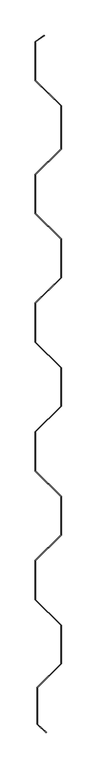
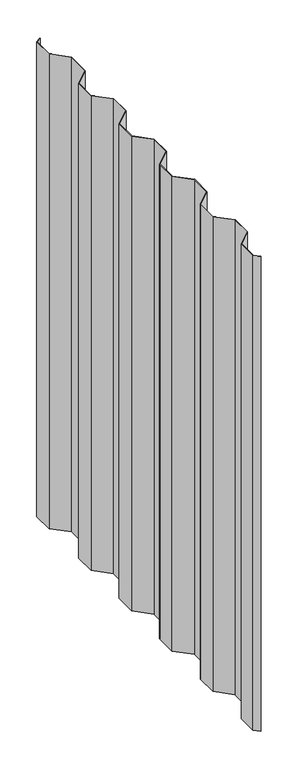
"""IFC4 building model written with IfcOpenShell, lengths in millimetres: proxy geometry, Generic Models 2:Generic Models 2:310765:Generic Models 2:310765 : Generic Models 2:Generic Models 2:310765:196 : Generic Models 2:Generic Models 2:310765:Generic Models 2:310765 : Generic Models 2:Generic Models 2:310765:300385."""

from ifc_helpers import new_model, si_unit, frame, origin, place, context, project, spatial, polyline, outline, extrude, source, transform, mapped, element, save


def generic_models_bcbc0872(model_context):
    return source(origin(), model_context, "Body", "SweptSolid", [
        extrude(outline(polyline([(579050.1098867, -578737.8387429), (579050.1098867, -578685.2449371), (579084.6679739, -578651.6129524), (579084.6679739, -578597.1045524), (579047.3617239, -578560.9423607), (579047.3617239, -578504.895144), (579084.6679739, -578468.7329524), (579084.6679739, -578414.2245524), (579047.3617239, -578378.0623607), (579047.3617239, -578322.015144), (579084.6679739, -578285.8529524), (579084.6679739, -578231.3445524), (579047.3617239, -578195.1823607), (579047.3617239, -578139.135144), (579084.6679739, -578102.9729524), (579084.6679739, -578048.4645524), (579047.3617239, -578012.3023607), (579047.3617239, -577956.255144), (579084.6679739, -577920.0929524), (579084.6679739, -577859.2345524), (579047.3617239, -577823.0723607), (579047.3617239, -577767.7945524), (579060.4697949, -577758.6161822), (579060.9250712, -577759.2663842), (579048.1554739, -577768.2077525), (579048.1554739, -577822.7363152), (579085.4617239, -577858.8985069), (579085.4617239, -577920.4289979), (579048.1554739, -577956.5911896), (579048.1554739, -578011.9663152), (579085.4617239, -578048.1285069), (579085.4617239, -578103.3089979), (579048.1554739, -578139.4711896), (579048.1554739, -578194.8463152), (579085.4617239, -578231.0085069), (579085.4617239, -578286.1889979), (579048.1554739, -578322.3511896), (579048.1554739, -578377.7263152), (579085.4617239, -578413.8885069), (579085.4617239, -578469.0689979), (579048.1554739, -578505.2311896), (579048.1554739, -578560.6063152), (579085.4617239, -578596.7685069), (579085.4617239, -578651.9480667), (579050.9036367, -578685.5800515), (579050.9036367, -578737.4864055), (579063.7799295, -578749.1325174), (579063.2179577, -578749.6944892), (579050.1098867, -578737.8387429)])), frame((0.0, 0.0, 4828.849258), z_axis=(0.0, 0.0, 1.0), x_axis=(1.0, 0.0, 0.0)), (0.0, 0.0, 1.0), 1305.250742),
    ])


if __name__ == "__main__":
    model = new_model("IFC4")
    model_context = context("Model", 3, world=origin())
    ifc_project = project(units=[si_unit("LENGTHUNIT", "METRE", prefix="MILLI")], contexts=[model_context])
    site = spatial("IfcSite", under=ifc_project)
    building = spatial("IfcBuilding", under=site)
    placement = place(None, origin())
    generic_models_shape = generic_models_bcbc0872(model_context)
    element("IfcBuildingElementProxy", 1, Name="Generic Models 2:Generic Models 2:310765:Generic Models 2:310765 : Generic Models 2:Generic Models 2:310765:196 : Generic Models 2:Generic Models 2:310765:Generic Models 2:310765 : Generic Models 2:Generic Models 2:310765:300385", ObjectType="Generic Models 2:Generic Models 2:310765:Generic Models 2:310765 : Generic Models 2:Generic Models 2:310765:196 : Generic Models 2:Generic Models 2:310765:Generic Models 2:310765 : Generic Models 2:Generic Models 2:310765:300385", at=placement, inside=building, context=model_context, shape_type="MappedRepresentation", body=[
        mapped(generic_models_shape, transform((0.0, 0.0, 0.0), x_axis=(1.0, 0.0, 0.0), y_axis=(0.0, 1.0, 0.0), z_axis=(0.0, 0.0, 1.0))),
    ])
    save(model, "model.ifc")

# Revit data of these elements
# Type "Generic Models 2:Generic Models 2:310765:Generic Models 2:310765 : Generic Models 2:Generic Models 2:310765:196 : Generic Models 2:Generic Models 2:310765:Generic Models 2:310765 : Generic Models 2:Generic Models 2:310765:300385"
#   NameOverride = "Generic Models 2:Generic Models 2:310765:Generic Models 2:310765 : Generic Models 2:Generic Models 2:310765:300385"
#   ObjectTypeOverride = "Generic Models 2:310765 : Generic Models 2:Generic Models 2:310765"
#   Reference = "Generic Models 2"
#   Tag = "300385"
# Element 1 (IfcBuildingElementProxy, "Generic Models 2:Generic Models 2:310765:Generic Models 2:310765 : Generic Models 2:Generic Models 2:310765:196 : Generic Models 2:Generic Models 2:310765:Generic Models 2:310765 : Generic Models 2:Generic Models 2:310765:300385")
#   Materials on its faces: "VERTICAL CORRUGATED METAL PANEL - EXPOSED FASTENERS - (MBCI 7.2 PANEL)"
# Materials
#   "VERTICAL CORRUGATED METAL PANEL - EXPOSED FASTENERS - (MBCI 7.2 PANEL)": class "Generic", colour RGB 120 120 120, transparency 0, Cost = 0
